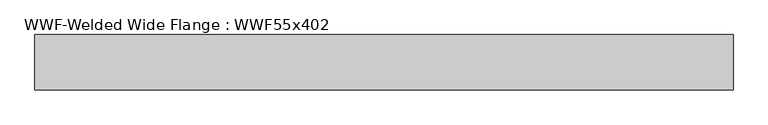
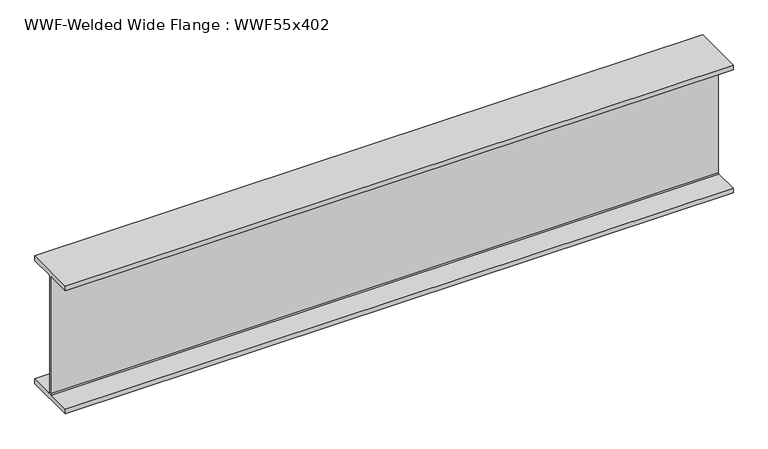
"""IFC4 building model written with IfcOpenShell, lengths in millimetres: beam geometry, WWF-Welded Wide Flange : WWF55x402."""

from ifc_helpers import new_model, si_unit, frame, origin, place, context, project, spatial, polyline, outline, extrude, source, transform, mapped, element, save


def wwf_welded_wide_flange_wwf55x402_a9ee8206(model_context):
    return source(origin(), model_context, "Body", "SweptSolid", [
        extrude(outline(polyline([(274.955, -649.986), (274.955, -700.024), (-274.955, -700.024), (-274.955, -649.986), (-19.05, -649.986), (-8.001, -638.937), (-8.001, 638.937), (-19.05, 649.986), (-274.955, 649.986), (-274.955, 700.024), (274.955, 700.024), (274.955, 649.986), (19.05, 649.986), (8.001, 638.937), (8.001, -638.937), (19.05, -649.986), (274.955, -649.986)])), frame((-3459.5263379, 0.0, 0.0), z_axis=(1.0, 0.0, 0.0), x_axis=(0.0, 1.0, 0.0)), (0.0, 0.0, 1.0), 6931.7526763),
    ])


if __name__ == "__main__":
    model = new_model("IFC4")
    model_context = context("Model", 3, world=origin())
    ifc_project = project(units=[si_unit("LENGTHUNIT", "METRE", prefix="MILLI")], contexts=[model_context])
    site = spatial("IfcSite", under=ifc_project)
    building = spatial("IfcBuilding", under=site)
    placement = place(None, origin())
    wwf_welded_wide_flange_wwf55x402_shape = wwf_welded_wide_flange_wwf55x402_a9ee8206(model_context)
    element("IfcBeam", 1, ObjectType="WWF-Welded Wide Flange : WWF55x402", at=placement, inside=building, context=model_context, shape_type="MappedRepresentation", body=[
        mapped(wwf_welded_wide_flange_wwf55x402_shape, transform((0.0, 0.0, 0.0), x_axis=(1.0, 0.0, 0.0), y_axis=(0.0, 1.0, 0.0), z_axis=(0.0, 0.0, 1.0))),
    ])
    save(model, "model.ifc")

# Revit data of these elements
# Type "WWF-Welded Wide Flange : WWF55x402"
#   Assembly Code = "B10"
#   Nominal d = "12"
#   W = 402
#   Length [instance default] = 1524 mm
#   bf = 549.91 mm
#   d = 1400.048 mm
#   k = 19.05 mm
#   tf = 50.038 mm
#   tw = 16.002 mm
#   A = 0.0761289 m²
#   Structural Material [instance default] = Steel ASTM A572
# Element 1 (IfcBeam, "WWF-Welded Wide Flange : WWF55x402")
#   Structural Material = Metal - Steel 43-275
#   Materials on its faces: "Metal - Steel 43-275"
# Materials
#   "Steel ASTM A572": class "Metal", colour RGB 247 247 247, transparency 0, Description = "Structural steel, high strength low alloy, ASTM - A572 - 50", Cost = 0
#   "Metal - Steel 43-275": class "Metal", colour RGB 247 247 247, transparency 0, Cost = 0
